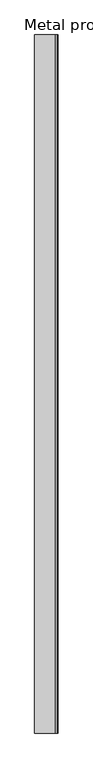
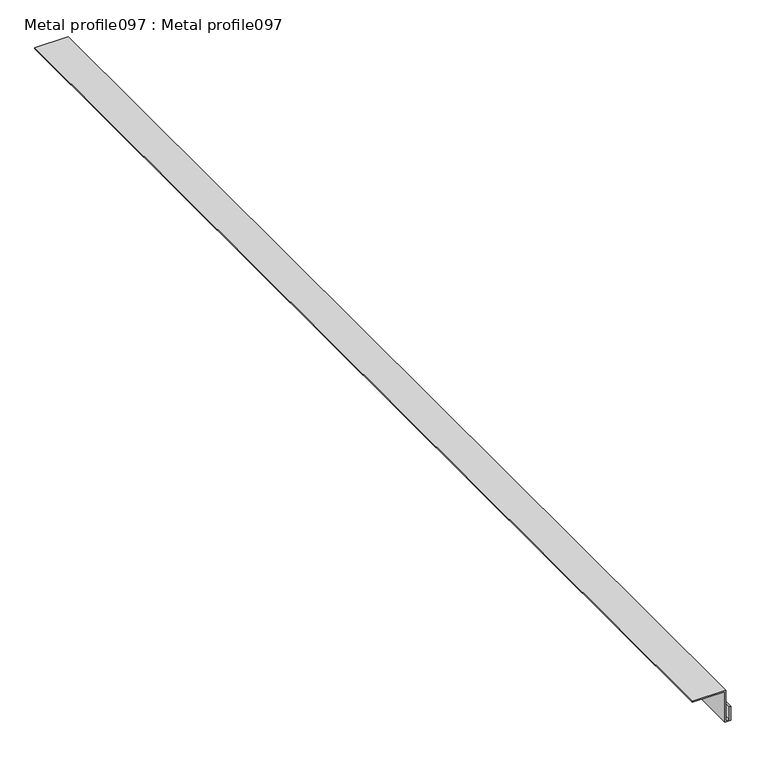
"""IFC4 building model written with IfcOpenShell, lengths in millimetres: proxy geometry, Metal profile097 : Metal profile097."""

from ifc_helpers import new_model, si_unit, frame, origin, place, context, project, spatial, polyline, outline, extrude, source, transform, mapped, element, save


def metal_profile097_metal_profile097_1ea8be3a(model_context):
    return source(origin(), model_context, "Body", "SweptSolid", [
        extrude(outline(polyline([(43467.2962907, 17693.9766245), (43493.6712907, 17693.9766245), (43493.6712907, 17691.9766245), (43469.2962907, 17691.9766245), (43469.2962907, 17685.5132456), (43526.4056657, 17685.5132456), (43526.4056657, 17626.8369761), (43524.4056657, 17626.8369761), (43524.4056657, 17683.5132456), (43467.2962907, 17683.5132456), (43467.2962907, 17693.9766245)])), frame((0.0, 7982.1507711, 0.0), z_axis=(0.0, 1.0, 0.0), x_axis=(0.0, 0.0, 1.0)), (0.0, 0.0, 1.0), 2000.0),
    ])


if __name__ == "__main__":
    model = new_model("IFC4")
    model_context = context("Model", 3, world=origin())
    ifc_project = project(units=[si_unit("LENGTHUNIT", "METRE", prefix="MILLI")], contexts=[model_context])
    site = spatial("IfcSite", under=ifc_project)
    building = spatial("IfcBuilding", under=site)
    placement = place(None, origin())
    metal_profile097_metal_profile097_shape = metal_profile097_metal_profile097_1ea8be3a(model_context)
    element("IfcBuildingElementProxy", 1, Name="Metal profile097 : Metal profile097", ObjectType="Metal profile097 : Metal profile097", at=placement, inside=building, context=model_context, shape_type="MappedRepresentation", body=[
        mapped(metal_profile097_metal_profile097_shape, transform((0.0, 0.0, 0.0), x_axis=(1.0, 0.0, 0.0), y_axis=(0.0, 1.0, 0.0), z_axis=(0.0, 0.0, 1.0))),
    ])
    save(model, "model.ifc")

# Revit data of these elements
# Type "Metal profile097 : Metal profile097"
#   NameOverride = "Metal profile097"
# Element 1 (IfcBuildingElementProxy, "Metal profile097 : Metal profile097")
#   Materials on its faces: "ANGLE TRIM 1419"
# Materials
#   "ANGLE TRIM 1419": class "Unassigned", colour RGB 250 255 0, transparency 0
